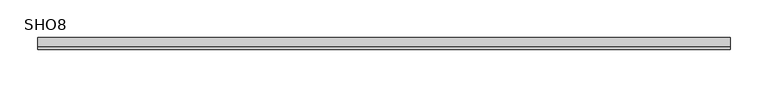
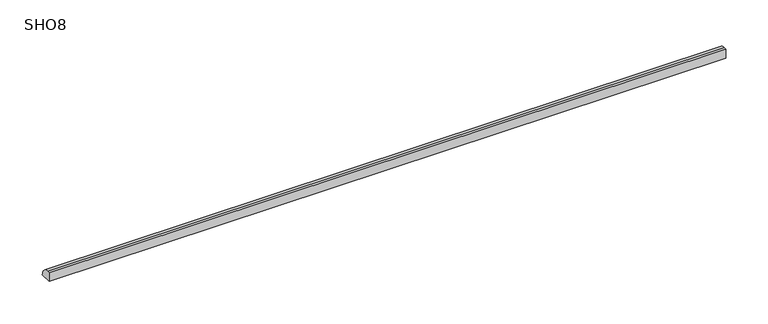
"""IFC4 building model written with IfcOpenShell, lengths in millimetres: proxy geometry, Molding-Merillat-Shoe : SHO8."""

from ifc_helpers import new_model, si_unit, point, frame, frame_2d, origin, place, context, project, spatial, polyline, circle_curve, trimmed, segment, composite_curve, outline, extrude, source, transform, mapped, element, save


def sho8_c9f749ba(model_context):
    return source(origin(), model_context, "Body", "SweptSolid", [
        extrude(outline(composite_curve([segment(polyline([(-15.875, 0.0), (-15.875, 12.7), (-12.7, 12.7)]), True, "CONTINUOUS"), segment(trimmed(circle_curve(frame_2d((-12.7, 0.0)), 12.7), [point((-12.7, 12.7))], [point((0.0, 0.0))], False, "CARTESIAN"), True, "CONTINUOUS"), segment(polyline([(0.0, 0.0), (-15.875, 0.0)]), True, "CONTINUOUS")], self_intersect=False)), frame((0.0, 0.0, 0.0), z_axis=(1.0, 0.0, 0.0), x_axis=(0.0, 1.0, 0.0)), (0.0, 0.0, 1.0), 919.1625),
    ])


if __name__ == "__main__":
    model = new_model("IFC4")
    model_context = context("Model", 3, world=origin())
    ifc_project = project(units=[si_unit("LENGTHUNIT", "METRE", prefix="MILLI")], contexts=[model_context])
    site = spatial("IfcSite", under=ifc_project)
    building = spatial("IfcBuilding", under=site)
    placement = place(None, origin())
    sho8_shape = sho8_c9f749ba(model_context)
    element("IfcBuildingElementProxy", 1, Name="Molding-Merillat-Shoe : SHO8", ObjectType="Molding-Merillat-Shoe : SHO8", at=placement, inside=building, context=model_context, shape_type="MappedRepresentation", body=[
        mapped(sho8_shape, transform((0.0, 0.0, 0.0), x_axis=(1.0, 0.0, 0.0), y_axis=(0.0, 1.0, 0.0), z_axis=(0.0, 0.0, 1.0))),
    ])
    save(model, "model.ifc")

# Revit data of these elements
# Type "Molding-Merillat-Shoe : SHO8"
#   URL = "http://www.merillat.com/"
#   Product Page URL = "http://www.merillat.com/our-products/rooms/kitchen/"
#   Product Documentation Link = "http://merillatbusiness.com/wp-content/uploads/2014/07/Merillat_Classic_Catalog.pdf"
#   Model = "SHO8"
#   Manufacturer = "Merillat"
#   Description = "Molding"
#   Construction Notes = "Available in 8' Individual Sections or Cartons of 25 (SHO8-25)"
#   Assembly Code = "C3010130"
#   Width [instance default] = 1' - 0"
#   Height = 0' - 0 5/8"
#   Depth = 0' - 0 1/2"
#   Default Elevation = 4' - 0"
#   COBie.Type = no
#   Straight [instance default] = yes
#   Right Outside Corner [instance default] = no
#   Right Inside Corner [instance default] = no
#   Left Outside Corner [instance default] = no
#   Left Inside Corner [instance default] = no
#   Molding Material = Wood - Merillat - Hazelnut
#   Type Comments = ""
# Element 1 (IfcBuildingElementProxy, "Molding-Merillat-Shoe : SHO8")
#   Width = 3' - 0 3/16"
#   Materials on its faces: "Wood - Merillat - Hazelnut"
# Materials
#   "Wood - Merillat - Hazelnut": class "Wood", colour RGB 138 103 81, transparency 0, Cost = 0
